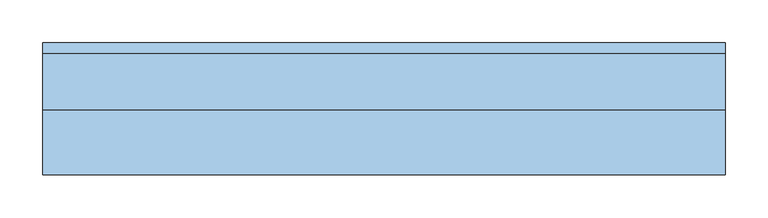
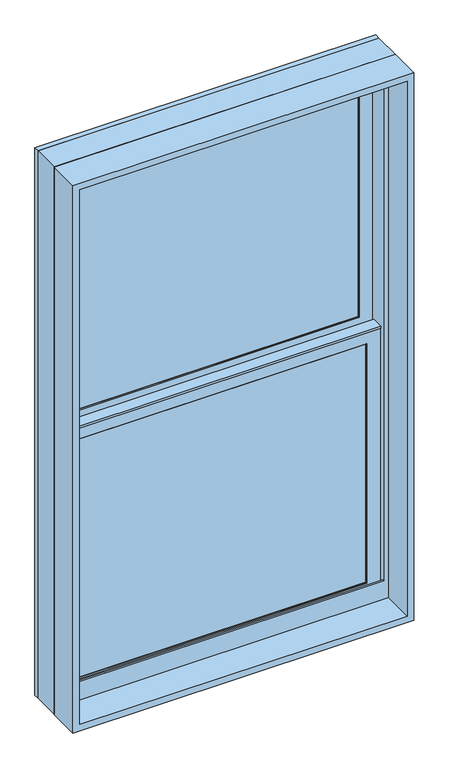
"""IFC4 building model written with IfcOpenShell, lengths in millimetres: window geometry, Window-Double_Hung-Marvin-Essential : ESDH2846."""

from ifc_helpers import new_model, si_unit, frame, origin, place, context, project, spatial, polyline, outline, extrude, faceted_brep, source, transform, mapped, element, save


def window_07479777(model_context):
    return source(origin(), model_context, "Body", "SolidModel", [
        extrude(outline(polyline([(123.825, 20.6375), (123.825, 15.875), (104.775, 15.875), (104.775, 20.6375), (123.825, 20.6375)])), frame((0.0, 0.0, 1136.65), z_axis=(0.0, 0.0, 1.0), x_axis=(1.0, 0.0, 0.0)), (0.0, 0.0, 1.0), 603.25),
        extrude(outline(polyline([(-104.775, 20.6375), (-104.775, 15.875), (-123.825, 15.875), (-123.825, 20.6375), (-104.775, 20.6375)])), frame((0.0, 0.0, 1136.65), z_axis=(0.0, 0.0, 1.0), x_axis=(1.0, 0.0, 0.0)), (0.0, 0.0, 1.0), 603.25),
        extrude(outline(polyline([(342.9, 20.6375), (342.9, 15.875), (-342.9, 15.875), (-342.9, 20.6375), (342.9, 20.6375)])), frame((0.0, 0.0, 1428.75), z_axis=(0.0, 0.0, 1.0), x_axis=(1.0, 0.0, 0.0)), (0.0, 0.0, 1.0), 19.05),
        extrude(outline(polyline([(-123.825, 46.83125), (-123.825, 51.59375), (-104.775, 51.59375), (-104.775, 46.83125), (-123.825, 46.83125)])), frame((0.0, 0.0, 1778.0), z_axis=(0.0, 0.0, 1.0), x_axis=(1.0, 0.0, 0.0)), (0.0, 0.0, 1.0), 603.25),
        extrude(outline(polyline([(104.775, 46.83125), (104.775, 51.59375), (123.825, 51.59375), (123.825, 46.83125), (104.775, 46.83125)])), frame((0.0, 0.0, 1778.0), z_axis=(0.0, 0.0, 1.0), x_axis=(1.0, 0.0, 0.0)), (0.0, 0.0, 1.0), 603.25),
        extrude(outline(polyline([(-342.9, 46.83125), (-342.9, 51.59375), (342.9, 51.59375), (342.9, 46.83125), (-342.9, 46.83125)])), frame((0.0, 0.0, 2070.1), z_axis=(0.0, 0.0, 1.0), x_axis=(1.0, 0.0, 0.0)), (0.0, 0.0, 1.0), 19.05),
        extrude(outline(polyline([(123.825, 20.6375), (104.775, 20.6375), (104.775, 25.4), (123.825, 25.4), (123.825, 20.6375)])), frame((0.0, 0.0, 1136.65), z_axis=(0.0, 0.0, 1.0), x_axis=(1.0, 0.0, 0.0)), (0.0, 0.0, 1.0), 603.25),
        extrude(outline(polyline([(-104.775, 20.6375), (-123.825, 20.6375), (-123.825, 25.4), (-104.775, 25.4), (-104.775, 20.6375)])), frame((0.0, 0.0, 1136.65), z_axis=(0.0, 0.0, 1.0), x_axis=(1.0, 0.0, 0.0)), (0.0, 0.0, 1.0), 603.25),
        extrude(outline(polyline([(342.9, 20.6375), (-342.9, 20.6375), (-342.9, 25.4), (342.9, 25.4), (342.9, 20.6375)])), frame((0.0, 0.0, 1428.75), z_axis=(0.0, 0.0, 1.0), x_axis=(1.0, 0.0, 0.0)), (0.0, 0.0, 1.0), 19.05),
        extrude(outline(polyline([(-123.825, 56.35625), (-104.775, 56.35625), (-104.775, 51.59375), (-123.825, 51.59375), (-123.825, 56.35625)])), frame((0.0, 0.0, 1778.0), z_axis=(0.0, 0.0, 1.0), x_axis=(1.0, 0.0, 0.0)), (0.0, 0.0, 1.0), 603.25),
        extrude(outline(polyline([(104.775, 56.35625), (123.825, 56.35625), (123.825, 51.59375), (104.775, 51.59375), (104.775, 56.35625)])), frame((0.0, 0.0, 1778.0), z_axis=(0.0, 0.0, 1.0), x_axis=(1.0, 0.0, 0.0)), (0.0, 0.0, 1.0), 603.25),
        extrude(outline(polyline([(-342.9, 56.35625), (342.9, 56.35625), (342.9, 51.59375), (-342.9, 51.59375), (-342.9, 56.35625)])), frame((0.0, 0.0, 2070.1), z_axis=(0.0, 0.0, 1.0), x_axis=(1.0, 0.0, 0.0)), (0.0, 0.0, 1.0), 19.05),
        faceted_brep([(-369.8875, 5.6780605, 1769.9351748), (-369.8875, 5.6780605, 1765.3), (369.8875, 5.6780605, 1765.3), (369.8875, 5.6780605, 1769.9351748), (-369.8875, 34.8118605, 1769.9351748), (369.8875, 34.8118605, 1769.9351748), (369.8875, 34.8118605, 1765.3), (-369.8875, 34.8118605, 1765.3), (-369.8875, 30.1625, 1765.3), (-369.8875, 30.1625, 1109.6625), (-369.8875, 8.9241104, 1109.6625), (-369.8875, 8.9241104, 1765.3), (369.8875, 8.9241104, 1765.3), (369.8875, 30.1625, 1765.3), (369.8875, 8.9241104, 1109.6625), (369.8875, 30.1625, 1109.6625), (-354.0034752, 11.90625, 1751.0034752), (-354.0034752, 30.1625, 1751.0034752), (354.0034752, 30.1625, 1751.0034752), (354.0034752, 11.90625, 1751.0034752), (-337.34375, 10.4662439, 1734.34375), (-337.34375, 11.90625, 1734.34375), (337.34375, 11.90625, 1734.34375), (337.34375, 10.4662439, 1734.34375), (338.8858834, 8.9241104, 1735.8858834), (-338.8858834, 8.9241104, 1735.8858834), (354.0034752, 30.1625, 1125.5465248), (354.0034752, 11.90625, 1125.5465248), (337.34375, 11.90625, 1142.20625), (337.34375, 10.4662439, 1142.20625), (338.8858834, 8.9241104, 1140.6641166), (-354.0034752, 30.1625, 1125.5465248), (-354.0034752, 11.90625, 1125.5465248), (-337.34375, 11.90625, 1142.20625), (-337.34375, 10.4662439, 1142.20625), (-338.8858834, 8.9241104, 1140.6641166)], [[[0, 1, 2, 3]], [[4, 5, 6, 7]], [[1, 0, 4, 7, 8, 9, 10, 11]], [[2, 1, 11, 12]], [[7, 6, 13, 8]], [[3, 2, 12, 14, 15, 13, 6, 5]], [[0, 3, 5, 4]], [[16, 17, 18, 19]], [[20, 21, 22, 23]], [[20, 23, 24, 25]], [[19, 18, 26, 27]], [[23, 22, 28, 29]], [[24, 23, 29, 30]], [[27, 26, 31, 32]], [[29, 28, 33, 34]], [[30, 29, 34, 35]], [[15, 14, 10, 9]], [[15, 9, 8, 13], [18, 17, 31, 26]], [[17, 16, 32, 31]], [[16, 19, 27, 32], [22, 21, 33, 28]], [[21, 20, 34, 33]], [[20, 25, 35, 34]], [[10, 14, 12, 11], [25, 24, 30, 35]]]),
        extrude(outline(polyline([(38.5955581, 1751.0125), (33.5778968, 1751.0125), (33.5778968, 1752.6), (39.9405976, 1752.6), (39.9405976, 1751.0125), (61.515625, 1751.0125), (47.6307501, 1747.6975159), (38.5955581, 1747.6975159), (38.5955581, 1751.0125)])), frame((-369.8875, 0.0, 0.0), z_axis=(1.0, 0.0, 0.0), x_axis=(0.0, 1.0, 0.0)), (0.0, 0.0, 1.0), 739.775),
        faceted_brep([(400.05, 0.0, 1079.5), (400.05, 0.0, 2438.4), (-400.05, 0.0, 2438.4), (-400.05, 0.0, 1079.5), (373.85625, 0.0, 1140.61875), (-373.85625, 0.0, 1140.61875), (-373.85625, 0.0, 2412.20625), (373.85625, 0.0, 2412.20625), (373.85625, 3.96875, 1079.5), (-373.85625, 3.96875, 1079.5), (-373.85625, 3.96875, 1140.61875), (373.85625, 3.96875, 1140.61875), (-400.05, 65.6828125, 1079.5), (-373.85625, 65.6828125, 1079.5), (373.85625, 65.6828125, 1079.5), (400.05, 65.6828125, 1079.5), (-400.05, 65.6828125, 2438.4), (400.05, 65.6828125, 2438.4), (373.85625, 65.6828125, 2412.20625), (-373.85625, 65.6828125, 2412.20625)], [[[0, 1, 2, 3], [4, 5, 6, 7]], [[8, 9, 10, 11]], [[5, 4, 11, 10]], [[0, 3, 12, 13, 9, 8, 14, 15]], [[13, 12, 16, 17, 15, 14, 18, 19]], [[13, 19, 6, 5, 10, 9]], [[7, 6, 19, 18]], [[18, 14, 8, 11, 4, 7]], [[1, 0, 15, 17]], [[2, 1, 17, 16]], [[3, 2, 16, 12]]]),
        faceted_brep([(373.85625, 30.1625, 1758.95), (372.26875, 30.1625, 1758.95), (372.26875, 30.1625, 1103.8544613), (373.85625, 30.1625, 1103.8544613), (-372.26875, 30.1625, 1758.95), (-373.85625, 30.1625, 1758.95), (-373.85625, 30.1625, 1103.8544613), (-372.26875, 30.1625, 1103.8544613), (372.26875, 63.5, 1758.95), (373.85625, 63.5, 1758.95), (373.85625, 63.5, 1097.3743077), (372.26875, 63.5, 1097.3743077), (-373.85625, 63.5, 1758.95), (-372.26875, 63.5, 1758.95), (-372.26875, 63.5, 1097.3743077), (-373.85625, 63.5, 1097.3743077), (385.1108932, 3.96875, 1108.9460105), (385.1108932, 3.96875, 1079.5), (385.1108932, 65.6828125, 1079.5), (385.1108932, 65.6828125, 1096.950012), (-385.1108932, 3.96875, 1079.5), (-385.1108932, 3.96875, 1108.9460105), (-385.1108932, 65.6828125, 1096.950012), (-385.1108932, 65.6828125, 1079.5), (385.1108932, 78.58125, 1094.4428097), (-385.1108932, 78.58125, 1094.4428097), (-383.0971252, 68.2348864, 1096.4539391), (-365.13135, 68.2348864, 1096.4539391), (-365.13135, 65.6828125, 1096.950012), (365.13135, 65.6828125, 1096.950012), (365.13135, 68.2348864, 1096.4539391), (383.0971252, 68.2348864, 1096.4539391), (-400.05, 65.6828125, 1079.5), (-400.05, 78.5948249, 1079.5), (400.05, 78.5948249, 1079.5), (400.05, 65.6828125, 1079.5), (-400.05, 78.58125, 2438.4), (400.05, 78.58125, 2438.4), (385.1108932, 78.58125, 2423.4608932), (-385.1108932, 78.58125, 2423.4608932), (-400.05, 65.6828125, 2438.4), (-383.0971252, 68.2348864, 2421.4471252), (383.0971252, 68.2348864, 2421.4471252), (365.13135, 68.2348864, 2403.48135), (-365.13135, 68.2348864, 2403.48135), (-365.13135, 65.6828125, 2403.48135), (365.13135, 65.6828125, 2403.48135), (400.05, 65.6828125, 2438.4)], [[[0, 1, 2, 3]], [[4, 5, 6, 7]], [[8, 9, 10, 11]], [[12, 13, 14, 15]], [[1, 8, 11, 2]], [[9, 0, 3, 10]], [[1, 0, 9, 8]], [[5, 4, 13, 12]], [[5, 12, 15, 6]], [[13, 4, 7, 14]], [[16, 17, 18, 19]], [[20, 21, 22, 23]], [[24, 25, 26, 27, 28, 22, 21, 16, 19, 29, 30, 31], [3, 2, 11, 10], [7, 6, 15, 14]], [[17, 16, 21, 20]], [[17, 20, 23, 32, 33, 34, 35, 18]], [[34, 33, 36, 37], [25, 24, 38, 39]], [[33, 32, 40, 36]], [[39, 41, 26, 25]], [[41, 42, 31, 30, 43, 44, 27, 26]], [[44, 45, 28, 27]], [[40, 32, 23, 22, 28, 45, 46, 29, 19, 18, 35, 47]], [[36, 40, 47, 37]], [[39, 38, 42, 41]], [[44, 43, 46, 45]], [[34, 37, 47, 35]], [[42, 38, 24, 31]], [[46, 43, 30, 29]]]),
        extrude(outline(polyline([(350.04375, 11.90625), (-350.04375, 11.90625), (-350.04375, 15.08125), (350.04375, 15.08125), (350.04375, 11.90625)])), frame((0.0, 0.0, 1129.50625), z_axis=(0.0, 0.0, 1.0), x_axis=(1.0, 0.0, 0.0)), (0.0, 0.0, 1.0), 617.5375),
        extrude(outline(polyline([(350.04375, 42.8625), (-350.04375, 42.8625), (-350.04375, 46.0375), (350.04375, 46.0375), (350.04375, 42.8625)])), frame((0.0, 0.0, 1770.85625), z_axis=(0.0, 0.0, 1.0), x_axis=(1.0, 0.0, 0.0)), (0.0, 0.0, 1.0), 617.5375),
        faceted_brep([(-337.34375, 31.194477, 1734.34375), (-338.8858834, 32.7366104, 1735.8858834), (338.8858834, 32.7366104, 1735.8858834), (337.34375, 31.194477, 1734.34375), (-337.34375, 30.1625, 1734.34375), (337.34375, 30.1625, 1734.34375), (-369.8875, 32.7366104, 1766.8875), (-369.8875, 30.1625, 1766.8875), (369.8875, 30.1625, 1766.8875), (369.8875, 32.7366104, 1766.8875), (338.8858834, 32.7366104, 1140.6641166), (337.34375, 31.194477, 1142.20625), (337.34375, 30.1625, 1142.20625), (369.8875, 30.1625, 1109.6625), (369.8875, 32.7366104, 1109.6625), (-338.8858834, 32.7366104, 1140.6641166), (-337.34375, 31.194477, 1142.20625), (-337.34375, 30.1625, 1142.20625), (-369.8875, 30.1625, 1109.6625), (-369.8875, 32.7366104, 1109.6625)], [[[0, 1, 2, 3]], [[4, 0, 3, 5]], [[6, 7, 8, 9]], [[3, 2, 10, 11]], [[5, 3, 11, 12]], [[9, 8, 13, 14]], [[11, 10, 15, 16]], [[12, 11, 16, 17]], [[14, 13, 18, 19]], [[9, 14, 19, 6], [1, 15, 10, 2]], [[16, 15, 1, 0]], [[17, 16, 0, 4]], [[7, 18, 13, 8], [5, 12, 17, 4]], [[19, 18, 7, 6]]]),
        faceted_brep([(-354.0034752, 42.8625, 2392.3534752), (-354.0034752, 61.11875, 2392.3534752), (354.0034752, 61.11875, 2392.3534752), (354.0034752, 42.8625, 2392.3534752), (-337.34375, 41.4224939, 2375.69375), (-337.34375, 42.8625, 2375.69375), (337.34375, 42.8625, 2375.69375), (337.34375, 41.4224939, 2375.69375), (-338.8858834, 39.8803604, 2377.2358834), (338.8858834, 39.8803604, 2377.2358834), (-369.8875, 61.11875, 2408.2375), (-369.8875, 39.8803604, 2408.2375), (369.8875, 39.8803604, 2408.2375), (369.8875, 61.11875, 2408.2375), (354.0034752, 61.11875, 1766.8965248), (354.0034752, 42.8625, 1766.8965248), (337.34375, 42.8625, 1783.55625), (337.34375, 41.4224939, 1783.55625), (338.8858834, 39.8803604, 1782.0141166), (369.8875, 39.8803604, 1751.0125), (369.8875, 61.11875, 1751.0125), (-354.0034752, 61.11875, 1766.8965248), (-354.0034752, 42.8625, 1766.8965248), (-337.34375, 42.8625, 1783.55625), (-337.34375, 41.4224939, 1783.55625), (-338.8858834, 39.8803604, 1782.0141166), (-369.8875, 39.8803604, 1751.0125), (-369.8875, 61.11875, 1751.0125)], [[[0, 1, 2, 3]], [[4, 5, 6, 7]], [[8, 4, 7, 9]], [[10, 11, 12, 13]], [[3, 2, 14, 15]], [[7, 6, 16, 17]], [[9, 7, 17, 18]], [[13, 12, 19, 20]], [[15, 14, 21, 22]], [[17, 16, 23, 24]], [[18, 17, 24, 25]], [[20, 19, 26, 27]], [[13, 20, 27, 10], [1, 21, 14, 2]], [[22, 21, 1, 0]], [[3, 15, 22, 0], [5, 23, 16, 6]], [[24, 23, 5, 4]], [[25, 24, 4, 8]], [[11, 26, 19, 12], [9, 18, 25, 8]], [[27, 26, 11, 10]]]),
        faceted_brep([(-369.8875, 61.11875, 1751.0125), (-369.8875, 63.6928604, 1751.0125), (369.8875, 63.6928604, 1751.0125), (369.8875, 61.11875, 1751.0125), (-337.34375, 62.150727, 1783.55625), (-337.34375, 61.11875, 1783.55625), (337.34375, 61.11875, 1783.55625), (337.34375, 62.150727, 1783.55625), (-338.8858834, 63.6928604, 1782.0141166), (338.8858834, 63.6928604, 1782.0141166), (369.8875, 63.6928604, 2408.2375), (369.8875, 61.11875, 2408.2375), (337.34375, 61.11875, 2375.69375), (337.34375, 62.150727, 2375.69375), (338.8858834, 63.6928604, 2377.2358834), (-369.8875, 63.6928604, 2408.2375), (-369.8875, 61.11875, 2408.2375), (-337.34375, 61.11875, 2375.69375), (-337.34375, 62.150727, 2375.69375), (-338.8858834, 63.6928604, 2377.2358834)], [[[0, 1, 2, 3]], [[4, 5, 6, 7]], [[8, 4, 7, 9]], [[3, 2, 10, 11]], [[7, 6, 12, 13]], [[9, 7, 13, 14]], [[11, 10, 15, 16]], [[13, 12, 17, 18]], [[14, 13, 18, 19]], [[16, 15, 1, 0]], [[3, 11, 16, 0], [5, 17, 12, 6]], [[18, 17, 5, 4]], [[19, 18, 4, 8]], [[1, 15, 10, 2], [9, 14, 19, 8]]]),
        extrude(outline(polyline([(350.04375, 26.19375), (-350.04375, 26.19375), (-350.04375, 30.1625), (350.04375, 30.1625), (350.04375, 26.19375)])), frame((0.0, 0.0, 1129.50625), z_axis=(0.0, 0.0, 1.0), x_axis=(1.0, 0.0, 0.0)), (0.0, 0.0, 1.0), 617.5375),
        extrude(outline(polyline([(350.04375, 57.15), (-350.04375, 57.15), (-350.04375, 61.11875), (350.04375, 61.11875), (350.04375, 57.15)])), frame((0.0, 0.0, 1770.85625), z_axis=(0.0, 0.0, 1.0), x_axis=(1.0, 0.0, 0.0)), (0.0, 0.0, 1.0), 617.5375),
        extrude(outline(polyline([(2438.4, 400.05), (2438.4, -400.05), (1079.5, -400.05), (1079.5, 400.05), (2438.4, 400.05)]), holes=[polyline([(2422.525, 384.175), (1095.375, 384.175), (1095.375, -384.175), (2422.525, -384.175), (2422.525, 384.175)])]), frame((0.0, -76.2, 0.0), z_axis=(0.0, 1.0, 0.0), x_axis=(0.0, 0.0, 1.0)), (0.0, 0.0, 1.0), 75.40625),
    ])


if __name__ == "__main__":
    model = new_model("IFC4")
    model_context = context("Model", 3, world=origin())
    ifc_project = project(units=[si_unit("LENGTHUNIT", "METRE", prefix="MILLI")], contexts=[model_context])
    site = spatial("IfcSite", under=ifc_project)
    building = spatial("IfcBuilding", under=site)
    placement = place(None, origin())
    window_shape = window_07479777(model_context)
    element("IfcWindow", 1, ObjectType="Window-Double_Hung-Marvin-Essential : ESDH2846", at=placement, inside=building, context=model_context, shape_type="MappedRepresentation", body=[
        mapped(window_shape, transform((0.0, 0.0, 0.0), x_axis=(1.0, 0.0, 0.0), y_axis=(0.0, 1.0, 0.0), z_axis=(0.0, 0.0, 1.0))),
    ])
    save(model, "model.ifc")

# Revit data of these elements
# Type "Window-Double_Hung-Marvin-Essential : ESDH2846"
#   Type Mark = "57"
#   Window Type = "Essential Double Hung"
#   Product data url = "https://bimobject.com/marvin-windows-and-doors/product/marvin-dhwau"
#   Product Guid = "c4a96547-874c-4385-91dc-a058adc19d98"
#   Frame = "All Ultrex"
#   Egress Window = "No"
#   URL = "www.marvin.com"
#   Model = "ESDH2846"
#   Manufacturer = "Marvin Windows and Doors"
#   Label Egress = ""
#   Glass Type = "IG Low E II with Argon"
#   Design Pressure = "DP50"
#   Description = "3254 DBHG"
#   Analytic Construction = "<None>"
#   Prairie Corner Width = 0' - 4"
#   Prairie Corner Height = 0' - 4"
#   Egress Width = 2' - 4 9/16"
#   Egress Height = 1' - 10 27/128"
#   Rough Width = 2' - 8"
#   Rough Height = 4' - 6"
#   Nominal Width = 2' - 8"
#   Nominal Height = 4' - 6"
#   Inset to Installation Flange [instance default] = 0' - 1"
#   Height = 4' - 5 1/2"
#   Egress Area = 4.40555 SF
#   Default Head Height = 8' - 0"
#   Width = 2' - 7 1/2"
#   Daylight Area = 8.60053 SF
#   DLO Width = 2' - 2 9/16"
#   DLO Height = 1' - 11 5/16"
#   Muntins Top Sash = yes
#   Lites Wide Top Sash = 3
#   Lites Wide Bottom Sash = 3
#   Lites High Top Sash = 2
#   Lites High Bottom Sash = 2
#   Lite Cut Prairie 9 = no
#   Lite Cut HV Grid = yes
#   Muntins Bottom Sash = yes
#   Label Visibility = no
#   Jamb Extension Visibility = yes
#   Edition number = 1
#   Interior Material = Ultrex-Marvin-Stonewhite
#   Glazing Material = Glass-Marvin-IG Low E II with Argon
#   Cladding Material = Ultrex-Marvin-Pebblegray
#   Wall Closure = (empty or 0)
#   Assembly Code = ""
# Element 1 (IfcWindow, "Window-Double_Hung-Marvin-Essential : ESDH2846")
#   Materials on its faces: "Ultrex-Marvin-Pebblegray", "Ultrex-Marvin-Stonewhite", "Glass-Marvin-IG Low E II with Argon"
# Materials
#   "Ultrex-Marvin-Stonewhite": class "Paint", colour RGB 250 251 245, transparency 0
#   "Glass-Marvin-IG Low E II with Argon": class "Glass", colour RGB 0 128 192, transparency 0.85
#   "Ultrex-Marvin-Pebblegray": class "Paint", colour RGB 189 185 173, transparency 0
